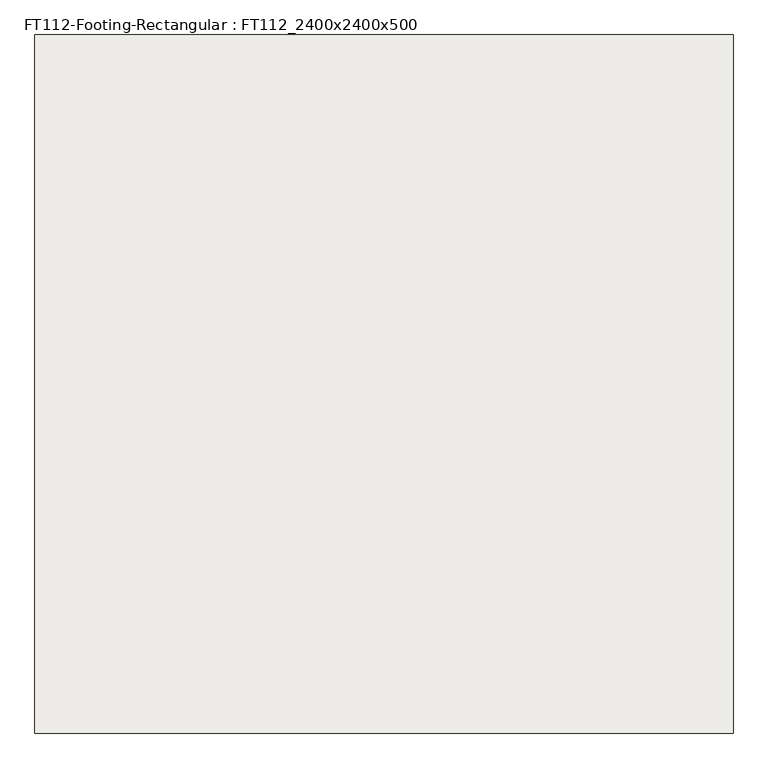
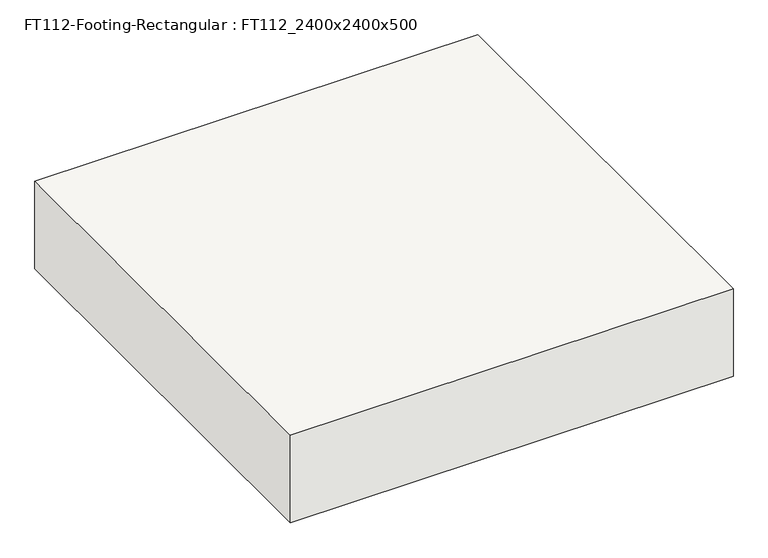
"""IFC4 building model written with IfcOpenShell, lengths in millimetres: slab geometry, FT112-Footing-Rectangular : FT112_2400x2400x500."""

from ifc_helpers import new_model, si_unit, frame, origin, place, context, project, spatial, polyline, outline, extrude, source, transform, mapped, element, save


def ft112_footing_rectangular_ft112_2400x2400x500_5fe39465(model_context):
    return source(origin(), model_context, "Body", "SweptSolid", [
        extrude(outline(polyline([(1200.0, 1200.0), (1200.0, -1200.0), (-1200.0, -1200.0), (-1200.0, 1200.0), (1200.0, 1200.0)])), frame((0.0, 0.0, -500.0), z_axis=(0.0, 0.0, 1.0), x_axis=(1.0, 0.0, 0.0)), (0.0, 0.0, 1.0), 500.0),
    ])


if __name__ == "__main__":
    model = new_model("IFC4")
    model_context = context("Model", 3, world=origin())
    ifc_project = project(units=[si_unit("LENGTHUNIT", "METRE", prefix="MILLI")], contexts=[model_context])
    site = spatial("IfcSite", under=ifc_project)
    building = spatial("IfcBuilding", under=site)
    placement = place(None, origin())
    ft112_footing_rectangular_ft112_2400x2400x500_shape = ft112_footing_rectangular_ft112_2400x2400x500_5fe39465(model_context)
    element("IfcSlab", 1, ObjectType="FT112-Footing-Rectangular : FT112_2400x2400x500", at=placement, inside=building, context=model_context, shape_type="MappedRepresentation", body=[
        mapped(ft112_footing_rectangular_ft112_2400x2400x500_shape, transform((0.0, 0.0, 0.0), x_axis=(1.0, 0.0, 0.0), y_axis=(0.0, 1.0, 0.0), z_axis=(0.0, 0.0, 1.0))),
    ])
    save(model, "model.ifc")

# Revit data of these elements
# Type "FT112-Footing-Rectangular : FT112_2400x2400x500"
#   Description = "UG Shallow Foundation"
#   Width = 2400 mm
#   Length = 2400 mm
#   Foundation Thickness = 500 mm
#   hec_material3 [instance default] = none
#   hec_material2 [instance default] = A03AE056-00001_Bitumen/Bituminous/Asphalt Coating
#   hec_material1 [instance default] = A03AC035-00001_Form Work (3 times in use)_Flat
#   Structural Material [instance default] = A03AC032-00007_Structural Concrete_Type1_25MPa-30Mpa
#   Assembly Code = ""
# Element 1 (IfcSlab, "FT112-Footing-Rectangular : FT112_2400x2400x500")
#   Structural Material = 콘크리트 - 현장타설 콘크리트
#   Materials on its faces: "콘크리트 - 현장타설 콘크리트"
# Materials
#   "A03AE056-00001_Bitumen/Bituminous/Asphalt Coating": class "Generic", colour RGB 17 17 17, transparency 0, Description = "Damp-proofing", W00) Work Master Code = "A03AE056-00001", W01) Work Master_Lv1 = "Concrete Work", W02) Work Master_Lv2 = "Concrete Protective Coating (U/G)", W03) Work Master_Spec.1 = "Bitumen/Bituminous/Asphalt Coating", Cost = 0
#   "A03AC035-00001_Form Work (3 times in use)_Flat": class "Wood", colour RGB 149 120 74, transparency 0, Description = "Plywood", W00) Work Master Code = "A03AC035-00001", W01) Work Master_Lv1 = "Concrete Work", W02) Work Master_Lv2 = "Substructure Work", W03) Work Master_Spec.1 = "Form Work (3 times in use)", W04) Work Master_Spec.2 = "Flat Form", W05) Work Master_Spec.3 = "Dressed Lumber, Plywood or Steel Form(Wood Planks are not Allowed) incl. Chamfer", Cost = 0
#   "A03AC032-00007_Structural Concrete_Type1_25MPa-30Mpa": class "Concrete", colour RGB 176 176 176, transparency 0, Keynote = "09910.A1", Description = "Reinf. Conc.", W00) Work Master Code = "A03AC032-00007", W01) Work Master_Lv1 = "Concrete Work", W02) Work Master_Lv2 = "Substructure Work", W03) Work Master_Spec.1 = "Structural Concrete", W04) Work Master_Spec.2 = "Cement Type-1", W05) Work Master_Spec.3 = "25MPa < F'c (Cylinder Strength) ≤ 30MPa", Cost = 0
#   "콘크리트 - 현장타설 콘크리트": class "콘크리트", colour RGB 192 192 192, transparency 0
